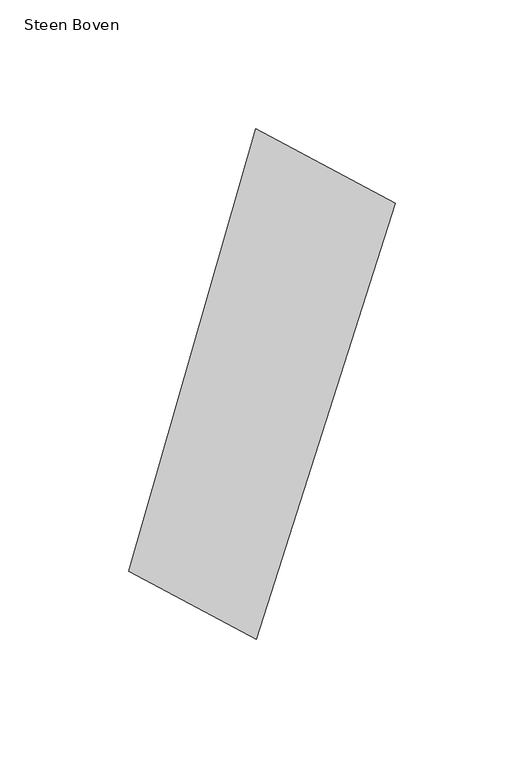
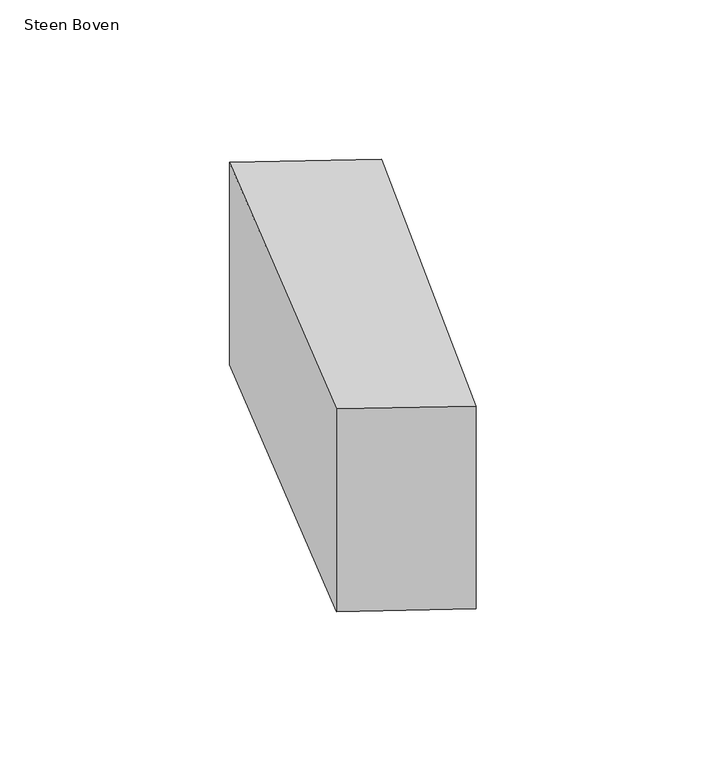
"""IFC4 building model written with IfcOpenShell, lengths in millimetres: proxy geometry, 00_GMA_steen_versie_4 : Steen Boven."""

from ifc_helpers import new_model, si_unit, origin, origin_with_axes, place, context, project, spatial, polyline, outline, extrude, source, transform, mapped, element, save


def steen_boven_cfa659d8(model_context):
    return source(origin(), model_context, "Body", "SweptSolid", [
        extrude(outline(polyline([(128.8449514, 158.2009929), (74.9550768, -11.5290371), (25.1908089, 15.0562908), (74.6750904, 187.1681388), (128.8449514, 158.2009929)])), origin_with_axes(), (0.0, 0.0, 1.0), 100.0),
    ])


if __name__ == "__main__":
    model = new_model("IFC4")
    model_context = context("Model", 3, world=origin())
    ifc_project = project(units=[si_unit("LENGTHUNIT", "METRE", prefix="MILLI")], contexts=[model_context])
    site = spatial("IfcSite", under=ifc_project)
    building = spatial("IfcBuilding", under=site)
    placement = place(None, origin())
    steen_boven_shape = steen_boven_cfa659d8(model_context)
    element("IfcBuildingElementProxy", 1, Name="00_GMA_steen_versie_4 : Steen Boven", ObjectType="00_GMA_steen_versie_4 : Steen Boven", at=placement, inside=building, context=model_context, shape_type="MappedRepresentation", body=[
        mapped(steen_boven_shape, transform((0.0, 0.0, 0.0), x_axis=(1.0, 0.0, 0.0), y_axis=(0.0, 1.0, 0.0), z_axis=(0.0, 0.0, 1.0))),
    ])
    save(model, "model.ifc")

# Revit data of these elements
# Type "00_GMA_steen_versie_4 : Steen Boven"
#   StootVoegHalfBoven [instance default] = 5 mm
#   StootVoegHalf [instance default] = 5 mm
#   StootVoegBreedteOnder = 10 mm
#   StootVoegBreedteBoven = 10 mm
#   Steendikte = 100 mm
#   LintVoegOnderHalf = 5 mm
#   LintVoegOnder = 10 mm
#   LintVoegBovenHalf = 0 mm
#   LintVoegBoven = 0 mm
#   materiaal = none
#   MateriaalVoeg = none
#   Default Elevation = 0
